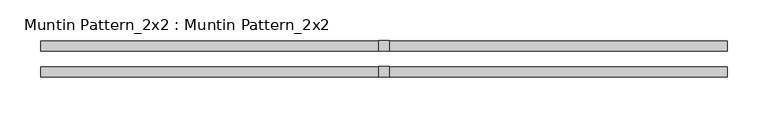
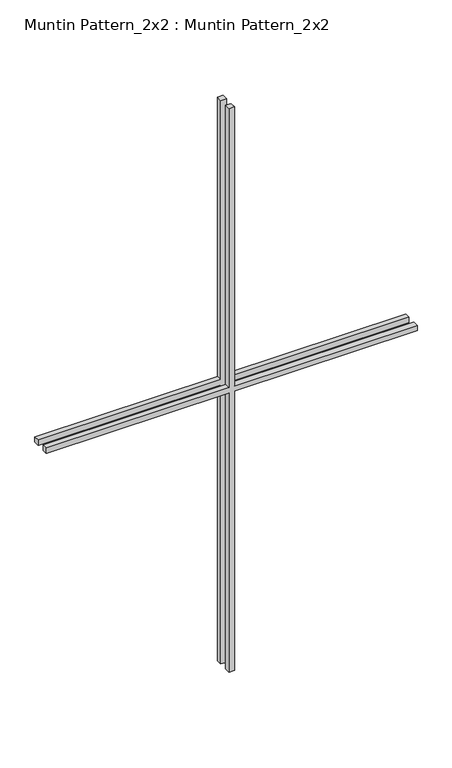
"""IFC4 building model written with IfcOpenShell, lengths in millimetres: proxy geometry, Muntin Pattern_2x2 : Muntin Pattern_2x2."""

from ifc_helpers import new_model, si_unit, frame, origin, place, context, project, spatial, polyline, outline, extrude, source, transform, mapped, element, save


def muntin_pattern_2x2_muntin_pattern_2x2_66e60b0d(model_context):
    return source(origin(), model_context, "Body", "SweptSolid", [
        extrude(outline(polyline([(679.45, -6.35), (679.45, -419.1), (666.75, -419.1), (666.75, -6.35), (0.0, -6.35), (0.0, 6.35), (666.75, 6.35), (666.75, 419.1), (679.45, 419.1), (679.45, 6.35), (1346.2, 6.35), (1346.2, -6.35), (679.45, -6.35)])), frame((0.0, 9.525, 0.0), z_axis=(0.0, 1.0, 0.0), x_axis=(0.0, 0.0, 1.0)), (0.0, 0.0, 1.0), 12.7),
        extrude(outline(polyline([(679.45, -6.35), (679.45, -419.1), (666.75, -419.1), (666.75, -6.35), (0.0, -6.35), (0.0, 6.35), (666.75, 6.35), (666.75, 419.1), (679.45, 419.1), (679.45, 6.35), (1346.2, 6.35), (1346.2, -6.35), (679.45, -6.35)])), frame((0.0, -22.225, 0.0), z_axis=(0.0, 1.0, 0.0), x_axis=(0.0, 0.0, 1.0)), (0.0, 0.0, 1.0), 12.7),
    ])


if __name__ == "__main__":
    model = new_model("IFC4")
    model_context = context("Model", 3, world=origin())
    ifc_project = project(units=[si_unit("LENGTHUNIT", "METRE", prefix="MILLI")], contexts=[model_context])
    site = spatial("IfcSite", under=ifc_project)
    building = spatial("IfcBuilding", under=site)
    placement = place(None, origin())
    muntin_pattern_2x2_muntin_pattern_2x2_shape = muntin_pattern_2x2_muntin_pattern_2x2_66e60b0d(model_context)
    element("IfcBuildingElementProxy", 1, Name="Muntin Pattern_2x2 : Muntin Pattern_2x2", ObjectType="Muntin Pattern_2x2 : Muntin Pattern_2x2", at=placement, inside=building, context=model_context, shape_type="MappedRepresentation", body=[
        mapped(muntin_pattern_2x2_muntin_pattern_2x2_shape, transform((0.0, 0.0, 0.0), x_axis=(1.0, 0.0, 0.0), y_axis=(0.0, 1.0, 0.0), z_axis=(0.0, 0.0, 1.0))),
    ])
    save(model, "model.ifc")

# Revit data of these elements
# Type "Muntin Pattern_2x2 : Muntin Pattern_2x2"
#   Width [instance default] = 4' - 0"
#   Thickness = 0' - 0 1/2"
#   Height [instance default] = 4' - 0"
#   Distance = 0' - 0 3/4"
#   Interior Material [instance default] = none
#   Exterior Material [instance default] = none
#   Default Elevation = 0
# Element 1 (IfcBuildingElementProxy, "Muntin Pattern_2x2 : Muntin Pattern_2x2")
#   Width = 2' - 9"
#   Height = 4' - 5"
#   Interior Material = Wood - Stained
#   Exterior Material = Clad - White
#   Materials on its faces: "Clad - White", "Wood - Stained"
# Materials
#   "Clad - White": class "Wood", colour RGB 242 242 238, transparency 0, Cost = 0
#   "Wood - Stained": class "Wood", colour RGB 224 178 126, transparency 0, Cost = 0
